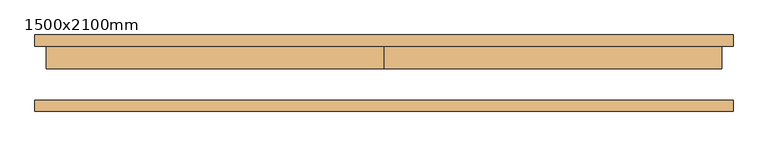
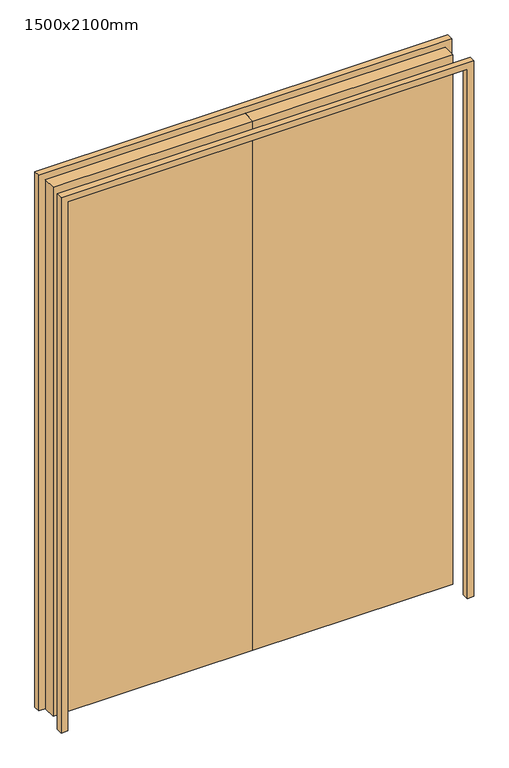
"""IFC4 building model written with IfcOpenShell, lengths in millimetres: door geometry, WWm-DoubleSolid-Flush : 1500x2100mm."""

import ifcopenshell
import ifcopenshell.guid

model = None  # the IFC model being written
_history = None  # IfcOwnerHistory: only IFC2X3 demands one
_inside = {}  # id of a spatial element -> (the spatial element, [elements in it])
_under = {}  # id of a project, library or spatial element -> (it, [spatial elements below it])
_declared = {}  # id of a project -> (the project, [libraries it declares])
_typed = {}  # id of a type object -> (the type object, [elements of that type])
_made_of = {}  # id of a material, layer set ... -> (it, [elements and type objects made of it])


def new_model(schema):
    """Start an empty IFC model of exactly this schema.

    Asked for "IFC4X3", IfcOpenShell would pick the latest addendum, in which some entities
    have other attributes; the version numbers below select the first issue.
    IFC2X3 requires an IfcOwnerHistory on every rooted entity: one is made here for all.
    """
    global model, _history
    if schema == "IFC4X3":
        model = ifcopenshell.file(schema_version=(4, 3, 0, 0))
    else:
        model = ifcopenshell.file(schema=schema)
    _inside.clear()
    _under.clear()
    _declared.clear()
    _typed.clear()
    _made_of.clear()
    _history = None
    if model.schema == "IFC2X3":
        org = make("IfcOrganization", Name="unknown")
        user = make(
            "IfcPersonAndOrganization",
            ThePerson=make("IfcPerson", FamilyName="unknown"),
            TheOrganization=org,
        )
        app = make(
            "IfcApplication",
            ApplicationDeveloper=org,
            Version="unknown",
            ApplicationFullName="unknown",
            ApplicationIdentifier="unknown",
        )
        _history = make(
            "IfcOwnerHistory",
            OwningUser=user,
            OwningApplication=app,
            ChangeAction="ADDED",
            CreationDate=0,
        )
    return model


def make(cls, **values):
    """One entity of the class cls with the attributes given. An attribute that is None is left unset."""
    return model.create_entity(
        cls, **{name: value for name, value in values.items() if value is not None}
    )


def rooted(cls, **values):
    """An entity with a GlobalId (a new one), such as an element, a storey or a relation."""
    return make(cls, GlobalId=ifcopenshell.guid.new(), OwnerHistory=_history, **values)


def si_unit(unit_type, name, prefix=None):
    """IfcSIUnit, for example si_unit("LENGTHUNIT", "METRE", prefix="MILLI")."""
    return make("IfcSIUnit", UnitType=unit_type, Prefix=prefix, Name=name)


def assignment(units):
    """IfcUnitAssignment: the units of a project."""
    return None if units is None else make("IfcUnitAssignment", Units=units)


def point(xyz):
    """IfcCartesianPoint."""
    return None if xyz is None else make("IfcCartesianPoint", Coordinates=xyz)


def direction(xyz):
    """IfcDirection."""
    return None if xyz is None else make("IfcDirection", DirectionRatios=xyz)


def frame(location, z_axis=None, x_axis=None):
    """IfcAxis2Placement3D, a coordinate frame: its origin and axes. An axis left out is left unset."""
    return make(
        "IfcAxis2Placement3D",
        Location=point(location),
        Axis=direction(z_axis),
        RefDirection=direction(x_axis),
    )


def origin():
    """The frame at (0, 0, 0) with its axes left unset."""
    return frame((0.0, 0.0, 0.0))


def origin_with_axes():
    """The frame at (0, 0, 0) with the z axis (0, 0, 1) and the x axis (1, 0, 0) written out."""
    return frame((0.0, 0.0, 0.0), z_axis=(0.0, 0.0, 1.0), x_axis=(1.0, 0.0, 0.0))


def place(relative_to, where):
    """IfcLocalPlacement: puts the frame where relative to a parent placement (None: the world)."""
    return make(
        "IfcLocalPlacement", PlacementRelTo=relative_to, RelativePlacement=where
    )


def context(
    kind, dimensions, precision=None, world=None, true_north=None, identifier=None
):
    """IfcGeometricRepresentationContext, for example the 3D "Model" context."""
    return make(
        "IfcGeometricRepresentationContext",
        ContextIdentifier=identifier,
        ContextType=kind,
        CoordinateSpaceDimension=dimensions,
        Precision=precision,
        WorldCoordinateSystem=world,
        TrueNorth=true_north,
    )


def project(units=None, contexts=None):
    """IfcProject with its units and contexts."""
    return rooted(
        "IfcProject",
        Name="project",
        RepresentationContexts=contexts,
        UnitsInContext=assignment(units),
    )


def spatial(cls, under=None, at=None, **own):
    """A site, building, storey or space (cls), placed at a placement, below another one or the project."""
    s = rooted(cls, ObjectPlacement=at, **own)
    if under is not None:
        _under.setdefault(under.id(), (under, []))[1].append(s)
    return s


def polyline(points):
    """IfcPolyline through the points."""
    return make("IfcPolyline", Points=[point(p) for p in points])


def outline(outer, holes=None, kind="AREA"):
    """IfcArbitraryClosedProfileDef: a profile drawn as a closed curve; with holes, ...WithVoids."""
    if holes is None:
        return make("IfcArbitraryClosedProfileDef", ProfileType=kind, OuterCurve=outer)
    return make(
        "IfcArbitraryProfileDefWithVoids",
        ProfileType=kind,
        OuterCurve=outer,
        InnerCurves=holes,
    )


def extrude(swept, where, along, depth):
    """IfcExtrudedAreaSolid: the profile swept, set in the frame where, extruded along a direction by depth."""
    return make(
        "IfcExtrudedAreaSolid",
        SweptArea=swept,
        Position=where,
        ExtrudedDirection=direction(along),
        Depth=depth,
    )


def shape(context_of_items, identifier, shape_type, items):
    """IfcShapeRepresentation: the items that make up one representation, for example the "Body"."""
    return make(
        "IfcShapeRepresentation",
        ContextOfItems=context_of_items,
        RepresentationIdentifier=identifier,
        RepresentationType=shape_type,
        Items=items,
    )


def source(mapping_origin, context_of_items, identifier, shape_type, items):
    """IfcRepresentationMap: a shape defined once, which mapped items show again and again."""
    return make(
        "IfcRepresentationMap",
        MappingOrigin=mapping_origin,
        MappedRepresentation=shape(context_of_items, identifier, shape_type, items),
    )


def transform(
    local_origin,
    x_axis=None,
    y_axis=None,
    z_axis=None,
    scale=None,
    scale2=None,
    scale3=None,
    uniform=True,
):
    """IfcCartesianTransformationOperator3D, or its non-uniform kind. x_axis, y_axis, z_axis: its Axis1, 2, 3."""
    if uniform:
        return make(
            "IfcCartesianTransformationOperator3D",
            Axis1=direction(x_axis),
            Axis2=direction(y_axis),
            LocalOrigin=point(local_origin),
            Scale=scale,
            Axis3=direction(z_axis),
        )
    return make(
        "IfcCartesianTransformationOperator3DnonUniform",
        Axis1=direction(x_axis),
        Axis2=direction(y_axis),
        LocalOrigin=point(local_origin),
        Scale=scale,
        Axis3=direction(z_axis),
        Scale2=scale2,
        Scale3=scale3,
    )


def mapped(mapping_source, mapping_target):
    """IfcMappedItem: shows the shape of a source again, moved by a transform."""
    return make(
        "IfcMappedItem", MappingSource=mapping_source, MappingTarget=mapping_target
    )


def made_of(thing, what):
    """Note that an element or type object is made of a material, layer set ...; save() writes the relation."""
    if what is not None:
        _made_of.setdefault(what.id(), (what, []))[1].append(thing)
    return thing


def element(
    cls,
    number,
    at=None,
    inside=None,
    cuts=None,
    type_object=None,
    material=None,
    context=None,
    identifier="Body",
    shape_type=None,
    held_by="IfcProductDefinitionShape",
    body=None,
    shapes=None,
    **own,
):
    """One element of the class cls, such as IfcWall. Its Tag is "e" and its number.

    at: its placement. inside: the storey or other place that contains it. cuts: it is an
    opening in that element (IfcRelVoidsElement). A single representation is given by context,
    identifier, shape_type and body (its items); several are given by shapes. held_by: the class
    of the entity that holds the representations. save() writes the other relations.
    """
    e = rooted(cls, Tag="e%d" % number, ObjectPlacement=at, **own)
    if body is not None:
        shapes = [shape(context, identifier, shape_type, body)]
    if shapes is not None:
        e.Representation = make(held_by, Representations=shapes)
    if inside is not None:
        _inside.setdefault(inside.id(), (inside, []))[1].append(e)
    if cuts is not None:
        rooted(
            "IfcRelVoidsElement", RelatingBuildingElement=cuts, RelatedOpeningElement=e
        )
    if type_object is not None:
        _typed.setdefault(type_object.id(), (type_object, []))[1].append(e)
    return made_of(e, material)


def aggregate(whole, parts):
    """IfcRelAggregates: a whole, such as a stair, and the parts it consists of."""
    return rooted("IfcRelAggregates", RelatingObject=whole, RelatedObjects=parts)


def save(model, path):
    """Write the relations noted so far, then the file.

    IfcRelAggregates (storeys below a building ...), IfcRelContainedInSpatialStructure (elements
    in a storey), IfcRelDefinesByType, IfcRelAssociatesMaterial and IfcRelDeclares: one each for
    every whole, place, type object, material and project.
    """
    for whole, parts in _under.values():
        aggregate(whole, parts)
    for where, things in _inside.values():
        rooted(
            "IfcRelContainedInSpatialStructure",
            RelatedElements=things,
            RelatingStructure=where,
        )
    for kind, things in _typed.values():
        rooted("IfcRelDefinesByType", RelatedObjects=things, RelatingType=kind)
    for what, things in _made_of.values():
        rooted("IfcRelAssociatesMaterial", RelatedObjects=things, RelatingMaterial=what)
    for by, libraries in _declared.values():
        rooted("IfcRelDeclares", RelatingContext=by, RelatedDefinitions=libraries)
    model.write(path)


def door_1500x2100mm_ffbec9ef(model_context):
    return source(origin(), model_context, "Body", "SweptSolid", [
        extrude(outline(polyline([(0.0, 60.0), (750.0, 60.0), (750.0, 10.0), (0.0, 10.0), (0.0, 60.0)])), origin_with_axes(), (0.0, 0.0, 1.0), 2100.0),
        extrude(outline(polyline([(-750.0, 60.0), (0.0, 60.0), (0.0, 10.0), (-750.0, 10.0), (-750.0, 60.0)])), origin_with_axes(), (0.0, 0.0, 1.0), 2100.0),
        extrude(outline(polyline([(2100.0, -750.0), (2100.0, 750.0), (0.0, 750.0), (0.0, 775.0), (2125.0, 775.0), (2125.0, -775.0), (0.0, -775.0), (0.0, -750.0), (2100.0, -750.0)])), frame((0.0, -85.0, 0.0), z_axis=(0.0, 1.0, 0.0), x_axis=(0.0, 0.0, 1.0)), (0.0, 0.0, 1.0), 25.0),
        extrude(outline(polyline([(2100.0, -750.0), (2100.0, 750.0), (0.0, 750.0), (0.0, 775.0), (2125.0, 775.0), (2125.0, -775.0), (0.0, -775.0), (0.0, -750.0), (2100.0, -750.0)])), frame((0.0, 60.0, 0.0), z_axis=(0.0, 1.0, 0.0), x_axis=(0.0, 0.0, 1.0)), (0.0, 0.0, 1.0), 25.0),
    ])


if __name__ == "__main__":
    model = new_model("IFC4")
    model_context = context("Model", 3, world=origin())
    ifc_project = project(units=[si_unit("LENGTHUNIT", "METRE", prefix="MILLI")], contexts=[model_context])
    site = spatial("IfcSite", under=ifc_project)
    building = spatial("IfcBuilding", under=site)
    placement = place(None, origin())
    door_1500x2100mm_shape = door_1500x2100mm_ffbec9ef(model_context)
    element("IfcDoor", 1, ObjectType="WWm-DoubleSolid-Flush : 1500x2100mm", at=placement, inside=building, context=model_context, shape_type="MappedRepresentation", body=[
        mapped(door_1500x2100mm_shape, transform((0.0, 0.0, 0.0), x_axis=(1.0, 0.0, 0.0), y_axis=(0.0, 1.0, 0.0), z_axis=(0.0, 0.0, 1.0))),
    ])
    save(model, "model.ifc")

# Revit data of these elements
# Type "WWm-DoubleSolid-Flush : 1500x2100mm"
#   Type Mark = "EX1-56"
#   Construction Type Id = "MDOOR"
#   Assembly Code = "C1020"
#   Analytic Construction = "Metal"
#   Thickness = 50 mm
#   Thermal Resistance (R) = 0.270117 (m²·K)/W
#   Heat Transfer Coefficient (U) = 3.7021 W/(m²·K)
#   Height = 2100 mm
#   Trim Projection Ext = 25 mm
#   Trim Projection Int = 25 mm
#   Trim Width = 25 mm
#   Width = 1500 mm
#   Not 90 Degree [instance default] = no
#   90 Degree [instance default] = yes
#   Door Material = WW-EC-RGB-White
#   Frame Material = WW-EC-RGB-White
#   Visual Light Transmittance = 0
#   Solar Heat Gain Coefficient = 0
#   Function = (empty or 0)
#   Wall Closure = (empty or 0)
# Element 1 (IfcDoor, "WWm-DoubleSolid-Flush : 1500x2100mm")
#   Materials on its faces: "WW-EC-RGB-White"
# Materials
#   "WW-EC-RGB-White": class "Generic", colour RGB 255 255 255, transparency 0, Comments = "If region requests off-white, swith asset color to RGB 231-228-220", Description = "Generic Color", Cost = 0
